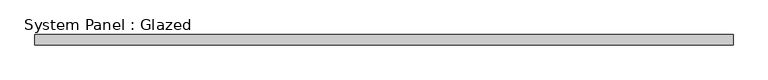
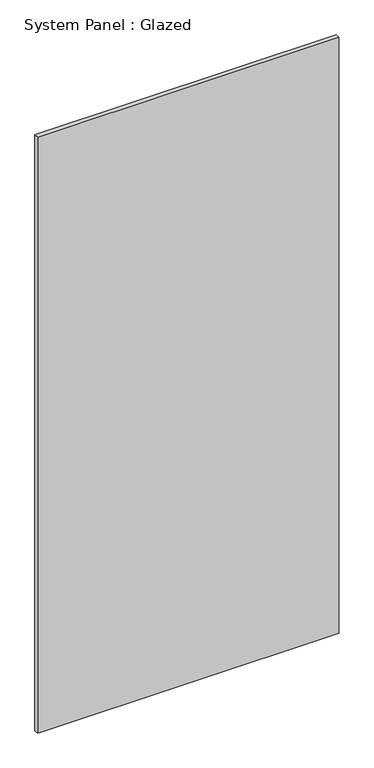
"""IFC4 building model written with IfcOpenShell, lengths in millimetres: plate geometry, System Panel : Glazed."""

import ifcopenshell
import ifcopenshell.guid

model = None  # the IFC model being written
_history = None  # IfcOwnerHistory: only IFC2X3 demands one
_inside = {}  # id of a spatial element -> (the spatial element, [elements in it])
_under = {}  # id of a project, library or spatial element -> (it, [spatial elements below it])
_declared = {}  # id of a project -> (the project, [libraries it declares])
_typed = {}  # id of a type object -> (the type object, [elements of that type])
_made_of = {}  # id of a material, layer set ... -> (it, [elements and type objects made of it])


def new_model(schema):
    """Start an empty IFC model of exactly this schema.

    Asked for "IFC4X3", IfcOpenShell would pick the latest addendum, in which some entities
    have other attributes; the version numbers below select the first issue.
    IFC2X3 requires an IfcOwnerHistory on every rooted entity: one is made here for all.
    """
    global model, _history
    if schema == "IFC4X3":
        model = ifcopenshell.file(schema_version=(4, 3, 0, 0))
    else:
        model = ifcopenshell.file(schema=schema)
    _inside.clear()
    _under.clear()
    _declared.clear()
    _typed.clear()
    _made_of.clear()
    _history = None
    if model.schema == "IFC2X3":
        org = make("IfcOrganization", Name="unknown")
        user = make(
            "IfcPersonAndOrganization",
            ThePerson=make("IfcPerson", FamilyName="unknown"),
            TheOrganization=org,
        )
        app = make(
            "IfcApplication",
            ApplicationDeveloper=org,
            Version="unknown",
            ApplicationFullName="unknown",
            ApplicationIdentifier="unknown",
        )
        _history = make(
            "IfcOwnerHistory",
            OwningUser=user,
            OwningApplication=app,
            ChangeAction="ADDED",
            CreationDate=0,
        )
    return model


def make(cls, **values):
    """One entity of the class cls with the attributes given. An attribute that is None is left unset."""
    return model.create_entity(
        cls, **{name: value for name, value in values.items() if value is not None}
    )


def rooted(cls, **values):
    """An entity with a GlobalId (a new one), such as an element, a storey or a relation."""
    return make(cls, GlobalId=ifcopenshell.guid.new(), OwnerHistory=_history, **values)


def si_unit(unit_type, name, prefix=None):
    """IfcSIUnit, for example si_unit("LENGTHUNIT", "METRE", prefix="MILLI")."""
    return make("IfcSIUnit", UnitType=unit_type, Prefix=prefix, Name=name)


def assignment(units):
    """IfcUnitAssignment: the units of a project."""
    return None if units is None else make("IfcUnitAssignment", Units=units)


def point(xyz):
    """IfcCartesianPoint."""
    return None if xyz is None else make("IfcCartesianPoint", Coordinates=xyz)


def direction(xyz):
    """IfcDirection."""
    return None if xyz is None else make("IfcDirection", DirectionRatios=xyz)


def frame(location, z_axis=None, x_axis=None):
    """IfcAxis2Placement3D, a coordinate frame: its origin and axes. An axis left out is left unset."""
    return make(
        "IfcAxis2Placement3D",
        Location=point(location),
        Axis=direction(z_axis),
        RefDirection=direction(x_axis),
    )


def origin():
    """The frame at (0, 0, 0) with its axes left unset."""
    return frame((0.0, 0.0, 0.0))


def origin_with_axes():
    """The frame at (0, 0, 0) with the z axis (0, 0, 1) and the x axis (1, 0, 0) written out."""
    return frame((0.0, 0.0, 0.0), z_axis=(0.0, 0.0, 1.0), x_axis=(1.0, 0.0, 0.0))


def place(relative_to, where):
    """IfcLocalPlacement: puts the frame where relative to a parent placement (None: the world)."""
    return make(
        "IfcLocalPlacement", PlacementRelTo=relative_to, RelativePlacement=where
    )


def context(
    kind, dimensions, precision=None, world=None, true_north=None, identifier=None
):
    """IfcGeometricRepresentationContext, for example the 3D "Model" context."""
    return make(
        "IfcGeometricRepresentationContext",
        ContextIdentifier=identifier,
        ContextType=kind,
        CoordinateSpaceDimension=dimensions,
        Precision=precision,
        WorldCoordinateSystem=world,
        TrueNorth=true_north,
    )


def project(units=None, contexts=None):
    """IfcProject with its units and contexts."""
    return rooted(
        "IfcProject",
        Name="project",
        RepresentationContexts=contexts,
        UnitsInContext=assignment(units),
    )


def spatial(cls, under=None, at=None, **own):
    """A site, building, storey or space (cls), placed at a placement, below another one or the project."""
    s = rooted(cls, ObjectPlacement=at, **own)
    if under is not None:
        _under.setdefault(under.id(), (under, []))[1].append(s)
    return s


def polyline(points):
    """IfcPolyline through the points."""
    return make("IfcPolyline", Points=[point(p) for p in points])


def outline(outer, holes=None, kind="AREA"):
    """IfcArbitraryClosedProfileDef: a profile drawn as a closed curve; with holes, ...WithVoids."""
    if holes is None:
        return make("IfcArbitraryClosedProfileDef", ProfileType=kind, OuterCurve=outer)
    return make(
        "IfcArbitraryProfileDefWithVoids",
        ProfileType=kind,
        OuterCurve=outer,
        InnerCurves=holes,
    )


def extrude(swept, where, along, depth):
    """IfcExtrudedAreaSolid: the profile swept, set in the frame where, extruded along a direction by depth."""
    return make(
        "IfcExtrudedAreaSolid",
        SweptArea=swept,
        Position=where,
        ExtrudedDirection=direction(along),
        Depth=depth,
    )


def shape(context_of_items, identifier, shape_type, items):
    """IfcShapeRepresentation: the items that make up one representation, for example the "Body"."""
    return make(
        "IfcShapeRepresentation",
        ContextOfItems=context_of_items,
        RepresentationIdentifier=identifier,
        RepresentationType=shape_type,
        Items=items,
    )


def source(mapping_origin, context_of_items, identifier, shape_type, items):
    """IfcRepresentationMap: a shape defined once, which mapped items show again and again."""
    return make(
        "IfcRepresentationMap",
        MappingOrigin=mapping_origin,
        MappedRepresentation=shape(context_of_items, identifier, shape_type, items),
    )


def transform(
    local_origin,
    x_axis=None,
    y_axis=None,
    z_axis=None,
    scale=None,
    scale2=None,
    scale3=None,
    uniform=True,
):
    """IfcCartesianTransformationOperator3D, or its non-uniform kind. x_axis, y_axis, z_axis: its Axis1, 2, 3."""
    if uniform:
        return make(
            "IfcCartesianTransformationOperator3D",
            Axis1=direction(x_axis),
            Axis2=direction(y_axis),
            LocalOrigin=point(local_origin),
            Scale=scale,
            Axis3=direction(z_axis),
        )
    return make(
        "IfcCartesianTransformationOperator3DnonUniform",
        Axis1=direction(x_axis),
        Axis2=direction(y_axis),
        LocalOrigin=point(local_origin),
        Scale=scale,
        Axis3=direction(z_axis),
        Scale2=scale2,
        Scale3=scale3,
    )


def mapped(mapping_source, mapping_target):
    """IfcMappedItem: shows the shape of a source again, moved by a transform."""
    return make(
        "IfcMappedItem", MappingSource=mapping_source, MappingTarget=mapping_target
    )


def made_of(thing, what):
    """Note that an element or type object is made of a material, layer set ...; save() writes the relation."""
    if what is not None:
        _made_of.setdefault(what.id(), (what, []))[1].append(thing)
    return thing


def element(
    cls,
    number,
    at=None,
    inside=None,
    cuts=None,
    type_object=None,
    material=None,
    context=None,
    identifier="Body",
    shape_type=None,
    held_by="IfcProductDefinitionShape",
    body=None,
    shapes=None,
    **own,
):
    """One element of the class cls, such as IfcWall. Its Tag is "e" and its number.

    at: its placement. inside: the storey or other place that contains it. cuts: it is an
    opening in that element (IfcRelVoidsElement). A single representation is given by context,
    identifier, shape_type and body (its items); several are given by shapes. held_by: the class
    of the entity that holds the representations. save() writes the other relations.
    """
    e = rooted(cls, Tag="e%d" % number, ObjectPlacement=at, **own)
    if body is not None:
        shapes = [shape(context, identifier, shape_type, body)]
    if shapes is not None:
        e.Representation = make(held_by, Representations=shapes)
    if inside is not None:
        _inside.setdefault(inside.id(), (inside, []))[1].append(e)
    if cuts is not None:
        rooted(
            "IfcRelVoidsElement", RelatingBuildingElement=cuts, RelatedOpeningElement=e
        )
    if type_object is not None:
        _typed.setdefault(type_object.id(), (type_object, []))[1].append(e)
    return made_of(e, material)


def aggregate(whole, parts):
    """IfcRelAggregates: a whole, such as a stair, and the parts it consists of."""
    return rooted("IfcRelAggregates", RelatingObject=whole, RelatedObjects=parts)


def save(model, path):
    """Write the relations noted so far, then the file.

    IfcRelAggregates (storeys below a building ...), IfcRelContainedInSpatialStructure (elements
    in a storey), IfcRelDefinesByType, IfcRelAssociatesMaterial and IfcRelDeclares: one each for
    every whole, place, type object, material and project.
    """
    for whole, parts in _under.values():
        aggregate(whole, parts)
    for where, things in _inside.values():
        rooted(
            "IfcRelContainedInSpatialStructure",
            RelatedElements=things,
            RelatingStructure=where,
        )
    for kind, things in _typed.values():
        rooted("IfcRelDefinesByType", RelatedObjects=things, RelatingType=kind)
    for what, things in _made_of.values():
        rooted("IfcRelAssociatesMaterial", RelatedObjects=things, RelatingMaterial=what)
    for by, libraries in _declared.values():
        rooted("IfcRelDeclares", RelatingContext=by, RelatedDefinitions=libraries)
    model.write(path)


def system_panel_glazed_e9b7a680(model_context):
    return source(origin(), model_context, "Body", "SweptSolid", [
        extrude(outline(polyline([(851.2699153, 19.05), (-851.2699153, 19.05), (-851.2699153, 44.45), (851.2699153, 44.45), (851.2699153, 19.05)])), origin_with_axes(), (0.0, 0.0, 1.0), 3562.35),
    ])


if __name__ == "__main__":
    model = new_model("IFC4")
    model_context = context("Model", 3, world=origin())
    ifc_project = project(units=[si_unit("LENGTHUNIT", "METRE", prefix="MILLI")], contexts=[model_context])
    site = spatial("IfcSite", under=ifc_project)
    building = spatial("IfcBuilding", under=site)
    placement = place(None, origin())
    system_panel_glazed_shape = system_panel_glazed_e9b7a680(model_context)
    element("IfcPlate", 1, ObjectType="System Panel : Glazed", at=placement, inside=building, context=model_context, shape_type="MappedRepresentation", body=[
        mapped(system_panel_glazed_shape, transform((0.0, 0.0, 0.0), x_axis=(1.0, 0.0, 0.0), y_axis=(0.0, 1.0, 0.0), z_axis=(0.0, 0.0, 1.0))),
    ])
    save(model, "model.ifc")

# Revit data of these elements
# Type "System Panel : Glazed"
#   Construction Type Id = "GSP4R"
#   Analytic Construction = "1/8 in Pilkington single glazing"
#   Visual Light Transmittance = 0.9
#   Solar Heat Gain Coefficient = 0.86
#   Heat Transfer Coefficient (U) = 1.18115 BTU/(h·ft²·°F)
#   Define Thermal Properties by = 1
# Element 1 (IfcPlate, "System Panel : Glazed")
#   Materials on its faces: "Glass"
# Materials
#   "Glass": class "Glass", colour RGB 0 128 192, transparency 0.75, Description = "Soda Lime Glass", Cost = 0
